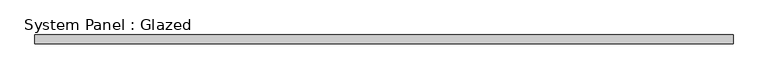
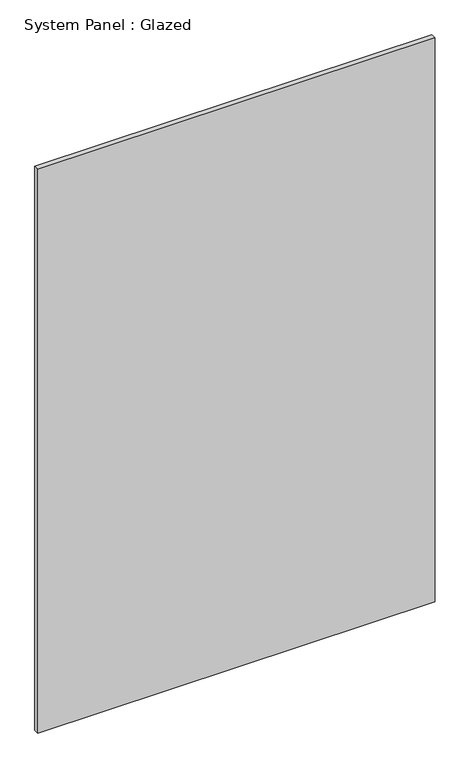
"""IFC4 building model written with IfcOpenShell, lengths in millimetres: plate geometry, System Panel : Glazed."""

from ifc_helpers import new_model, si_unit, origin, origin_with_axes, place, context, project, spatial, polyline, outline, extrude, source, transform, mapped, element, save


def system_panel_glazed_ecaba6c9(model_context):
    return source(origin(), model_context, "Body", "SweptSolid", [
        extrude(outline(polyline([(975.0, 24.5), (-975.0, 24.5), (-975.0, 49.5), (975.0, 49.5), (975.0, 24.5)])), origin_with_axes(), (0.0, 0.0, 1.0), 2925.0),
    ])


if __name__ == "__main__":
    model = new_model("IFC4")
    model_context = context("Model", 3, world=origin())
    ifc_project = project(units=[si_unit("LENGTHUNIT", "METRE", prefix="MILLI")], contexts=[model_context])
    site = spatial("IfcSite", under=ifc_project)
    building = spatial("IfcBuilding", under=site)
    placement = place(None, origin())
    system_panel_glazed_shape = system_panel_glazed_ecaba6c9(model_context)
    element("IfcPlate", 1, ObjectType="System Panel : Glazed", at=placement, inside=building, context=model_context, shape_type="MappedRepresentation", body=[
        mapped(system_panel_glazed_shape, transform((0.0, 0.0, 0.0), x_axis=(1.0, 0.0, 0.0), y_axis=(0.0, 1.0, 0.0), z_axis=(0.0, 0.0, 1.0))),
    ])
    save(model, "model.ifc")

# Revit data of these elements
# Element 1 (IfcPlate, "System Panel : Glazed")
#   Materials on its faces: "Glass"
# Materials
#   "Glass": class "Glass", colour RGB 0 128 192, transparency 0.9
